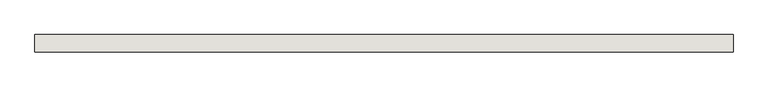
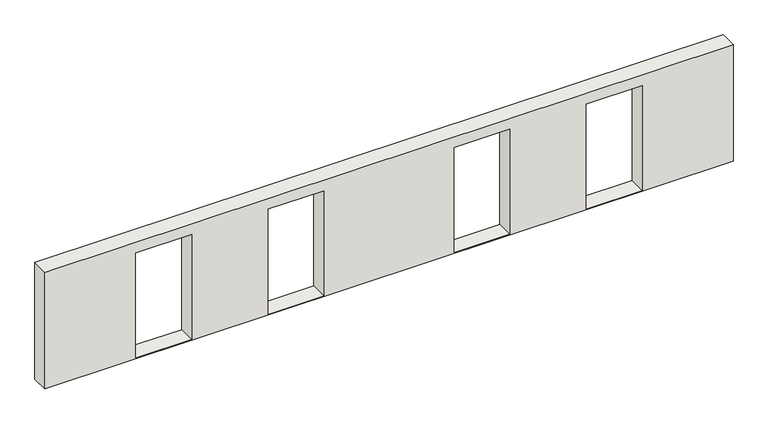
"""IFC4 building model written with IfcOpenShell, lengths in millimetres: wall geometry, 0_3d_modell."""

from ifc_helpers import new_model, si_unit, frame, origin, place, context, project, spatial, polyline, outline, extrude, source, transform, mapped, element, save


def wall_929ee36e(model_context):
    return source(origin(), model_context, "Body", "SweptSolid", [
        extrude(outline(polyline([(0.0, 0.0), (0.0, 14000.0), (2510.0, 14000.0), (2510.0, 0.0), (0.0, 0.0)]), holes=[polyline([(20.0, 11015.0), (2280.0, 11015.0), (2280.0, 12150.0), (20.0, 12150.0), (20.0, 11015.0)]), polyline([(20.0, 8325.0), (2280.0, 8325.0), (2280.0, 9460.0), (20.0, 9460.0), (20.0, 8325.0)]), polyline([(20.0, 4540.0), (2280.0, 4540.0), (2280.0, 5675.0), (20.0, 5675.0), (20.0, 4540.0)]), polyline([(20.0, 1850.0), (2280.0, 1850.0), (2280.0, 2985.0), (20.0, 2985.0), (20.0, 1850.0)])]), frame((0.0, 0.0, 0.0), z_axis=(0.0, 1.0, 0.0), x_axis=(0.0, 0.0, 1.0)), (0.0, 0.0, 1.0), 350.0),
    ])


if __name__ == "__main__":
    model = new_model("IFC4")
    model_context = context("Model", 3, world=origin())
    ifc_project = project(units=[si_unit("LENGTHUNIT", "METRE", prefix="MILLI")], contexts=[model_context])
    site = spatial("IfcSite", under=ifc_project)
    building = spatial("IfcBuilding", under=site)
    placement = place(None, origin())
    wall_shape = wall_929ee36e(model_context)
    element("IfcWall", 1, ObjectType="0_3d_modell", at=placement, inside=building, context=model_context, shape_type="MappedRepresentation", body=[
        mapped(wall_shape, transform((0.0, 0.0, 0.0), x_axis=(1.0, 0.0, 0.0), y_axis=(0.0, 1.0, 0.0), z_axis=(0.0, 0.0, 1.0))),
    ])
    save(model, "model.ifc")

# Revit data of these elements
# Element 1 (IfcWall, "0_3d_modell")
#   Materials on its faces: "holzschalung"
# Materials
#   "holzschalung": class "Unassigned", colour RGB 128 128 128, transparency 0
